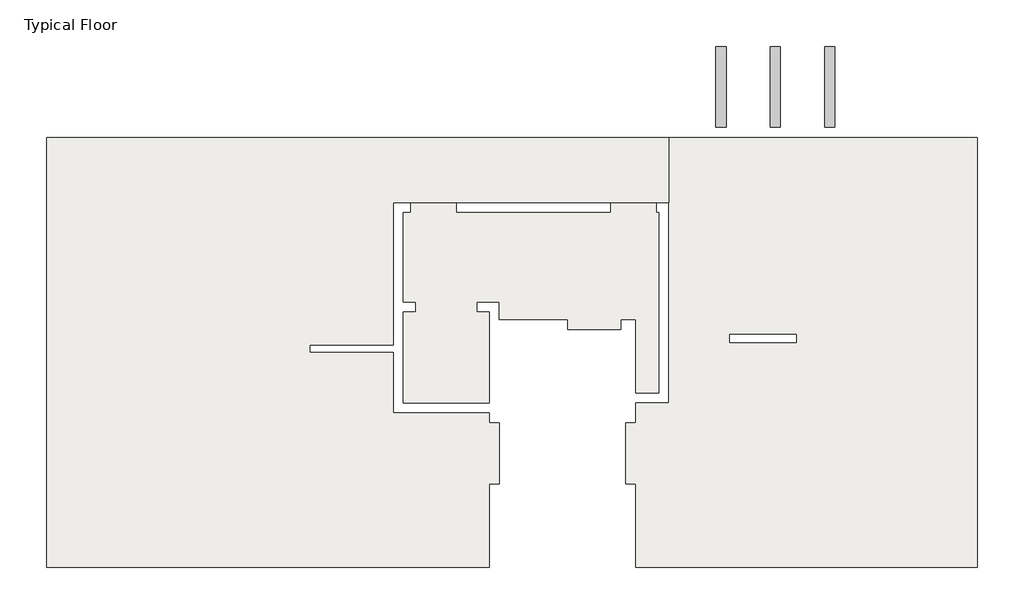
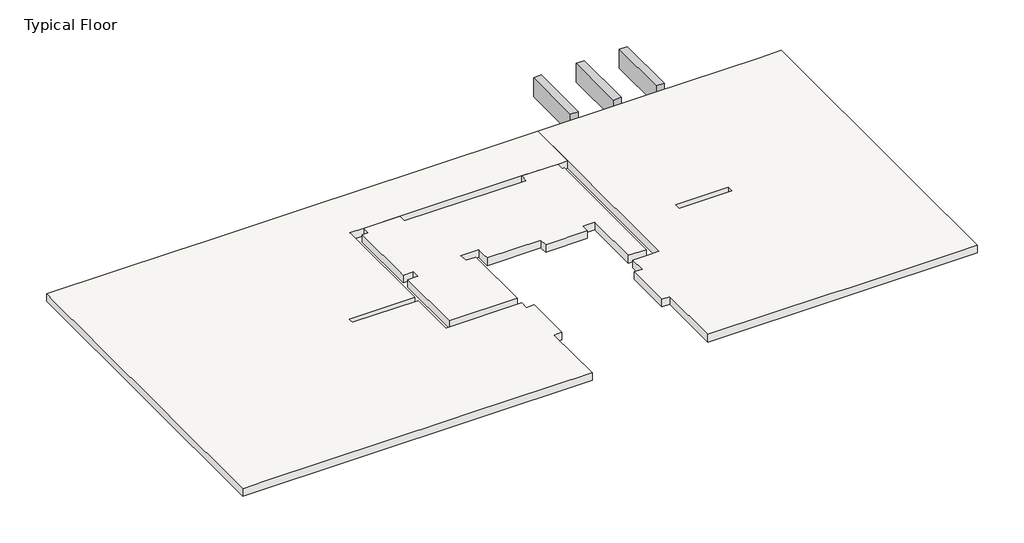
# One storey: 3 beams, 3 slabs.
"""IFC4 building model written with IfcOpenShell, lengths in millimetres."""

from ifc_helpers import new_model, si_unit, frame, origin, place, context, project, spatial, polyline, outline, extrude, faceted_brep, element, save

model = new_model("IFC4")

# Units and contexts
model_context = context("Model", 3, world=origin())
ifc_project = project(units=[si_unit("LENGTHUNIT", "METRE", prefix="MILLI")], contexts=[model_context])

# Site, building, storey
site = spatial("IfcSite", under=ifc_project)
building = spatial("IfcBuilding", under=site)
storey = spatial("IfcBuildingStorey", under=building, Name="Typical Floor", Elevation=3150.0)

# Beams
placement = place(None, origin())
element("IfcBeam", 1, ObjectType="Concrete Rectengular Beam : 20/50", at=placement, inside=storey, context=model_context, shape_type="SweptSolid", body=[
    extrude(outline(polyline([(-18417.3921114, 45934.7104697), (-18617.3921114, 45934.7104697), (-18617.3921114, 47534.7104697), (-18417.3921114, 47534.7104697), (-18417.3921114, 45934.7104697)])), frame((0.0, 0.0, 2650.0), z_axis=(0.0, 0.0, 1.0), x_axis=(1.0, 0.0, 0.0)), (0.0, 0.0, 1.0), 500.0),
])
element("IfcBeam", 2, ObjectType="Concrete Rectengular Beam : 20/50", at=placement, inside=storey, context=model_context, shape_type="Brep", body=[
    faceted_brep([(-19694.4921114, 45934.7104697, 3150.0), (-19587.9882316, 45934.7104697, 3150.0), (-19494.4921114, 45934.7104697, 3150.0), (-19494.4921114, 47534.7104697, 3150.0), (-19694.4921114, 47534.7104697, 3150.0), (-19694.4921114, 45934.7104697, 2650.0), (-19694.4921114, 47534.7104697, 2650.0), (-19494.4921114, 45934.7104697, 2650.0), (-19494.4921114, 47534.7104697, 2650.0)], [[[0, 1, 2, 3, 4]], [[5, 0, 4, 6]], [[7, 5, 6, 8]], [[2, 7, 8, 3]], [[4, 3, 8, 6]], [[2, 1, 0, 5, 7]]]),
])
element("IfcBeam", 3, ObjectType="Concrete Rectengular Beam : 20/50", at=placement, inside=storey, context=model_context, shape_type="SweptSolid", body=[
    extrude(outline(polyline([(-20566.8921114, 45934.7104697), (-20766.8921114, 45934.7104697), (-20766.8921114, 47534.7104697), (-20566.8921114, 47534.7104697), (-20566.8921114, 45934.7104697)])), frame((0.0, 0.0, 2650.0), z_axis=(0.0, 0.0, 1.0), x_axis=(1.0, 0.0, 0.0)), (0.0, 0.0, 1.0), 500.0),
])

# Slabs
element("IfcSlab", 4, ObjectType="20", at=placement, inside=storey, context=model_context, shape_type="Brep", body=[
    faceted_brep([(-25248.1921114, 38884.7104697, 2950.0), (-25248.1921114, 37234.7104697, 2950.0), (-33998.1921114, 37234.7104697, 2950.0), (-33998.1921114, 45734.7104697, 2950.0), (-21698.192111, 45734.7104697, 2950.0), (-21698.192111, 44444.7104697, 2950.0), (-21948.1921114, 44444.7104697, 2950.0), (-22848.1921114, 44444.7104697, 2950.0), (-25898.1921114, 44444.7104697, 2950.0), (-26798.1921114, 44444.7104697, 2950.0), (-27148.1921114, 44444.7104697, 2950.0), (-27148.1921114, 44244.7104697, 2950.0), (-27148.1921114, 41634.7104697, 2950.0), (-28798.1921114, 41634.7104697, 2950.0), (-28798.1921114, 41484.7104697, 2950.0), (-27148.1921114, 41484.7104697, 2950.0), (-27148.1921114, 40484.7104697, 2950.0), (-27148.1921114, 40284.7104697, 2950.0), (-25248.1921114, 40284.7104697, 2950.0), (-25248.1921114, 40084.7104697, 2950.0), (-25048.1921114, 40084.7104697, 2950.0), (-25048.1921114, 38884.7104697, 2950.0), (-25248.1921114, 37234.7104697, 3150.0), (-25248.1921114, 38884.7104697, 3150.0), (-25048.1921114, 38884.7104697, 3150.0), (-25048.1921114, 40084.7104697, 3150.0), (-25248.1921114, 40084.7104697, 3150.0), (-25248.1921114, 40284.7104697, 3150.0), (-27148.1921114, 40284.7104697, 3150.0), (-27148.1921114, 40484.7104697, 3150.0), (-27148.1921114, 41484.7104697, 3150.0), (-28798.1921114, 41484.7104697, 3150.0), (-28798.1921114, 41634.7104697, 3150.0), (-27148.1921114, 41634.7104697, 3150.0), (-27148.1921114, 44244.7104697, 3150.0), (-27148.1921114, 44444.7104697, 3150.0), (-26798.1921114, 44444.7104697, 3150.0), (-25898.1921114, 44444.7104697, 3150.0), (-22848.1921114, 44444.7104697, 3150.0), (-21948.1921114, 44444.7104697, 3150.0), (-21698.192111, 44444.7104697, 3150.0), (-21698.192111, 45734.7104697, 3150.0), (-22297.8129925, 45734.7104697, 3150.0), (-26418.1921114, 45734.7104697, 3150.0), (-27148.1921114, 45734.7104697, 3150.0), (-30003.1920714, 45734.7104697, 3150.0), (-30733.1920714, 45734.7104697, 3150.0), (-33998.1921114, 45734.7104697, 3150.0), (-33998.1921114, 45434.7104697, 3150.0), (-33998.1921114, 43778.8121651, 3150.0), (-33998.1921114, 43278.8121651, 3150.0), (-33998.1921114, 40884.7121321, 3150.0), (-33998.1921114, 40384.7121321, 3150.0), (-33998.1921114, 37234.7104697, 3150.0), (-33449.2609999, 37234.7104697, 3150.0), (-28799.0775982, 37234.7104697, 3150.0), (-28319.0775982, 37234.7104697, 3150.0)], [[[0, 1, 2, 3, 4, 5, 6, 7, 8, 9, 10, 11, 12, 13, 14, 15, 16, 17, 18, 19, 20, 21]], [[22, 23, 24, 25, 26, 27, 28, 29, 30, 31, 32, 33, 34, 35, 36, 37, 38, 39, 40, 41, 42, 43, 44, 45, 46, 47, 48, 49, 50, 51, 52, 53, 54, 55, 56]], [[1, 0, 23, 22]], [[2, 1, 22, 56, 55, 54, 53]], [[3, 2, 53, 52, 51, 50, 49, 48, 47]], [[4, 3, 47, 46, 45, 44, 43, 42, 41]], [[5, 4, 41, 40]], [[5, 40, 39, 38, 37, 36, 35, 10, 9, 8, 7, 6]], [[10, 35, 34, 33, 12, 11]], [[13, 12, 33, 32]], [[14, 13, 32, 31]], [[15, 14, 31, 30]], [[15, 30, 29, 28, 17, 16]], [[18, 17, 28, 27]], [[19, 18, 27, 26]], [[20, 19, 26, 25]], [[21, 20, 25, 24]], [[0, 21, 24, 23]]]),
])
element("IfcSlab", 5, ObjectType="20", at=placement, inside=storey, context=model_context, shape_type="Brep", body=[
    faceted_brep([(-26948.1921114, 40484.7104697, 2950.0), (-26948.1921114, 42284.7104697, 2950.0), (-26698.1921114, 42284.7104697, 2950.0), (-26698.1921114, 42484.7104697, 2950.0), (-26948.1921114, 42484.7104697, 2950.0), (-26948.1921114, 44244.7104697, 2950.0), (-26798.1921114, 44244.7104697, 2950.0), (-26798.1921114, 44444.7104697, 2950.0), (-25898.1921114, 44444.7104697, 2950.0), (-25898.1921114, 44244.7104697, 2950.0), (-22848.1921114, 44244.7104697, 2950.0), (-22848.1921114, 44444.7104697, 2950.0), (-21948.1921114, 44444.7104697, 2950.0), (-21948.1921114, 44244.7104697, 2950.0), (-21898.192111, 44244.7104697, 2950.0), (-21898.192111, 40684.7104697, 2950.0), (-22348.1921114, 40684.7104697, 2950.0), (-22348.1921114, 41934.7104698, 2950.0), (-22348.1921114, 42134.7104698, 2950.0), (-22648.1921114, 42134.7104698, 2950.0), (-22648.1921114, 41934.7104698, 2950.0), (-23698.1921114, 41934.7104698, 2950.0), (-23698.1921114, 42134.7104697, 2950.0), (-25048.1921114, 42134.7104697, 2950.0), (-25048.1921114, 42284.7104696, 2950.0), (-25048.1921114, 42484.7104696, 2950.0), (-25498.1921114, 42484.7104696, 2950.0), (-25498.1921114, 42284.7104696, 2950.0), (-25248.1921114, 42284.7104696, 2950.0), (-25248.1921114, 40484.7104697, 2950.0), (-26948.1921114, 42284.7104697, 3150.0), (-26948.1921114, 40484.7104697, 3150.0), (-25248.1921114, 40484.7104697, 3150.0), (-25248.1921114, 42284.7104696, 3150.0), (-25498.1921114, 42284.7104696, 3150.0), (-25498.1921114, 42484.7104696, 3150.0), (-25048.1921114, 42484.7104696, 3150.0), (-25048.1921114, 42284.7104696, 3150.0), (-25048.1921114, 42134.7104697, 3150.0), (-23698.1921114, 42134.7104697, 3150.0), (-23698.1921114, 41934.7104698, 3150.0), (-22648.1921114, 41934.7104698, 3150.0), (-22648.1921114, 42134.7104698, 3150.0), (-22348.1921114, 42134.7104698, 3150.0), (-22348.1921114, 41934.7104698, 3150.0), (-22348.1921114, 40684.7104697, 3150.0), (-21898.192111, 40684.7104697, 3150.0), (-21898.192111, 44244.7104697, 3150.0), (-21948.1921114, 44244.7104697, 3150.0), (-21948.1921114, 44444.7104697, 3150.0), (-22848.1921114, 44444.7104697, 3150.0), (-22848.1921114, 44244.7104697, 3150.0), (-25898.1921114, 44244.7104697, 3150.0), (-25898.1921114, 44444.7104697, 3150.0), (-26798.1921114, 44444.7104697, 3150.0), (-26798.1921114, 44244.7104697, 3150.0), (-26948.1921114, 44244.7104697, 3150.0), (-26948.1921114, 42484.7104697, 3150.0), (-26698.1921114, 42484.7104697, 3150.0), (-26698.1921114, 42284.7104697, 3150.0)], [[[0, 1, 2, 3, 4, 5, 6, 7, 8, 9, 10, 11, 12, 13, 14, 15, 16, 17, 18, 19, 20, 21, 22, 23, 24, 25, 26, 27, 28, 29]], [[30, 31, 32, 33, 34, 35, 36, 37, 38, 39, 40, 41, 42, 43, 44, 45, 46, 47, 48, 49, 50, 51, 52, 53, 54, 55, 56, 57, 58, 59]], [[1, 0, 31, 30]], [[2, 1, 30, 59]], [[3, 2, 59, 58]], [[4, 3, 58, 57]], [[5, 4, 57, 56]], [[6, 5, 56, 55]], [[7, 6, 55, 54]], [[8, 7, 54, 53]], [[9, 8, 53, 52]], [[10, 9, 52, 51]], [[11, 10, 51, 50]], [[12, 11, 50, 49]], [[13, 12, 49, 48]], [[14, 13, 48, 47]], [[15, 14, 47, 46]], [[16, 15, 46, 45]], [[16, 45, 44, 43, 18, 17]], [[19, 18, 43, 42]], [[20, 19, 42, 41]], [[21, 20, 41, 40]], [[22, 21, 40, 39]], [[23, 22, 39, 38]], [[23, 38, 37, 36, 25, 24]], [[26, 25, 36, 35]], [[27, 26, 35, 34]], [[28, 27, 34, 33]], [[29, 28, 33, 32]], [[0, 29, 32, 31]]]),
])
element("IfcSlab", 6, ObjectType="20", at=placement, inside=storey, context=model_context, shape_type="Brep", body=[
    faceted_brep([(-22548.1921114, 40084.7104697, 2950.0), (-22348.1921114, 40084.7104697, 2950.0), (-22348.1921114, 40484.7104697, 2950.0), (-21898.192111, 40484.7104697, 2950.0), (-21698.192111, 40484.7104697, 2950.0), (-21698.192111, 44244.7104697, 2950.0), (-21698.192111, 44444.7104697, 2950.0), (-21698.192111, 45734.7104697, 2950.0), (-15598.1921114, 45734.7104697, 2950.0), (-15598.1921114, 37234.7104697, 2950.0), (-22348.1921114, 37234.7104697, 2950.0), (-22348.1921114, 38884.7104697, 2950.0), (-22548.1921114, 38884.7104697, 2950.0), (-19178.1921114, 41834.7104349, 2950.0), (-20498.1921114, 41834.7104349, 2950.0), (-20498.1921114, 41684.7104349, 2950.0), (-19178.1921114, 41684.7104349, 2950.0), (-22348.1921114, 40084.7104697, 3150.0), (-22548.1921114, 40084.7104697, 3150.0), (-22548.1921114, 38884.7104697, 3150.0), (-22348.1921114, 38884.7104697, 3150.0), (-22348.1921114, 37234.7104697, 3150.0), (-19279.0292046, 37234.7104697, 3150.0), (-18799.0292046, 37234.7104697, 3150.0), (-16128.1921114, 37234.7104697, 3150.0), (-15598.1921114, 37234.7104697, 3150.0), (-15598.1921114, 39884.7076972, 3150.0), (-15598.1921114, 40384.7076972, 3150.0), (-15598.1921114, 45734.7104697, 3150.0), (-16128.1921114, 45734.7104697, 3150.0), (-18867.9882316, 45734.7104697, 3150.0), (-19587.9882316, 45734.7104697, 3150.0), (-21697.8129925, 45734.7104697, 3150.0), (-21698.192111, 45734.7104697, 3150.0), (-21698.192111, 44444.7104697, 3150.0), (-21698.192111, 44244.7104697, 3150.0), (-21698.192111, 40484.7104697, 3150.0), (-21898.192111, 40484.7104697, 3150.0), (-22348.1921114, 40484.7104697, 3150.0), (-20498.1921114, 41834.7104349, 3150.0), (-19178.1921114, 41834.7104349, 3150.0), (-19178.1921114, 41684.7104349, 3150.0), (-20498.1921114, 41684.7104349, 3150.0)], [[[0, 1, 2, 3, 4, 5, 6, 7, 8, 9, 10, 11, 12], [13, 14, 15, 16]], [[17, 18, 19, 20, 21, 22, 23, 24, 25, 26, 27, 28, 29, 30, 31, 32, 33, 34, 35, 36, 37, 38], [39, 40, 41, 42]], [[1, 0, 18, 17]], [[2, 1, 17, 38]], [[2, 38, 37, 36, 4, 3]], [[4, 36, 35, 34, 33, 7, 6, 5]], [[8, 7, 33, 32, 31, 30, 29, 28]], [[9, 8, 28, 27, 26, 25]], [[10, 9, 25, 24, 23, 22, 21]], [[11, 10, 21, 20]], [[12, 11, 20, 19]], [[0, 12, 19, 18]], [[14, 13, 40, 39]], [[15, 14, 39, 42]], [[16, 15, 42, 41]], [[13, 16, 41, 40]]]),
])

save(model, "model.ifc")

# Revit data of these elements
# Type "Concrete Rectengular Beam : 20/50"
#   Length [instance default] = 152.4 cm
#   b = 20 cm
#   h = 50 cm
#   Structural Material [instance default] = Concrete
#   Assembly Code = ""
# Type "20"
#   Function = 0
#   Layers, outside or top first: 20 cm "Concrete" (function 1)
# Element 1 (IfcBeam, "Concrete Rectengular Beam : 20/50")
#   Comments = ""
#   Mark = "B19"
#   SOFiSTiK_AMG_Comments = ""
#   SOFiSTiK_AMG_Scheduled = yes
#   SOFiSTiK_AMG_Adjusted = yes
#   Structural Material = Concrete
#   Phase Created = New Construction
#   Materials on its faces: "Concrete"
# Element 2 (IfcBeam, "Concrete Rectengular Beam : 20/50")
#   Comments = ""
#   Mark = "B20"
#   SOFiSTiK_AMG_Comments = ""
#   SOFiSTiK_AMG_Scheduled = yes
#   SOFiSTiK_AMG_Adjusted = yes
#   Structural Material = Concrete
#   Phase Created = New Construction
#   Materials on its faces: "Concrete"
# Element 3 (IfcBeam, "Concrete Rectengular Beam : 20/50")
#   Comments = ""
#   Mark = "B21"
#   SOFiSTiK_AMG_Comments = ""
#   SOFiSTiK_AMG_Scheduled = yes
#   SOFiSTiK_AMG_Adjusted = yes
#   Structural Material = Concrete
#   Phase Created = New Construction
#   Materials on its faces: "Concrete"
# Element 4 (IfcSlab, "20")
#   Mark = "S1"
#   SOFiSTiK_AMG_Comments = ""
#   built-in parameter 1001955 = 1.5708 (stored number, unit not read)
#   Height Offset From Level = 0 cm
#   built-in parameter 1001954 = 1
#   SOFiSTiK_AMG_Scheduled = yes
#   SOFiSTiK_AMG_Adjusted = yes
#   Phase Created = New Construction
#   Materials on its faces: "Concrete"
# Element 5 (IfcSlab, "20")
#   Mark = "S2"
#   SOFiSTiK_AMG_Comments = ""
#   built-in parameter 1001955 = 3.14159 (stored number, unit not read)
#   Height Offset From Level = 0 cm
#   built-in parameter 1001954 = 1
#   SOFiSTiK_AMG_Scheduled = yes
#   SOFiSTiK_AMG_Adjusted = yes
#   Phase Created = New Construction
#   Materials on its faces: "Concrete"
# Element 6 (IfcSlab, "20")
#   Mark = "S3"
#   SOFiSTiK_AMG_Comments = ""
#   built-in parameter 1001955 = 1.5708 (stored number, unit not read)
#   Height Offset From Level = 0 cm
#   built-in parameter 1001954 = 1
#   SOFiSTiK_AMG_Scheduled = yes
#   SOFiSTiK_AMG_Adjusted = yes
#   Phase Created = New Construction
#   Materials on its faces: "Concrete"
# Materials
#   "Concrete": class "Concrete", colour RGB 192 192 192, transparency 0, Keynote = "01000", Description = "Cast-in-place concrete", Cost = 0
